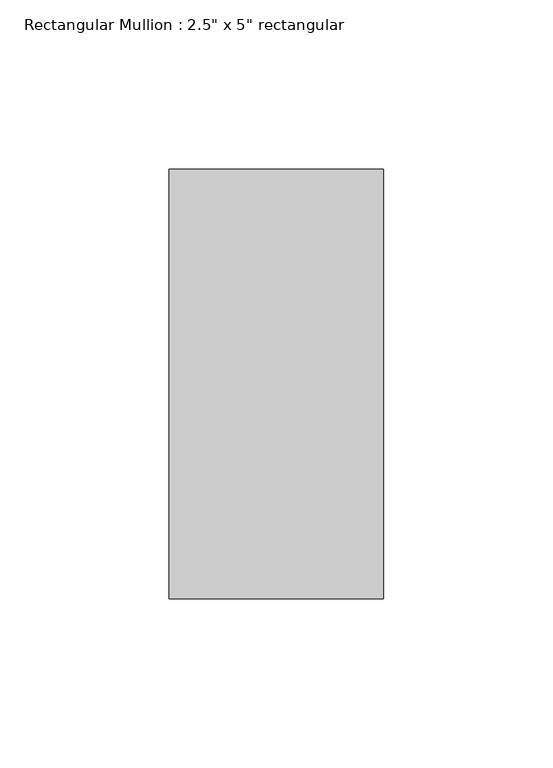
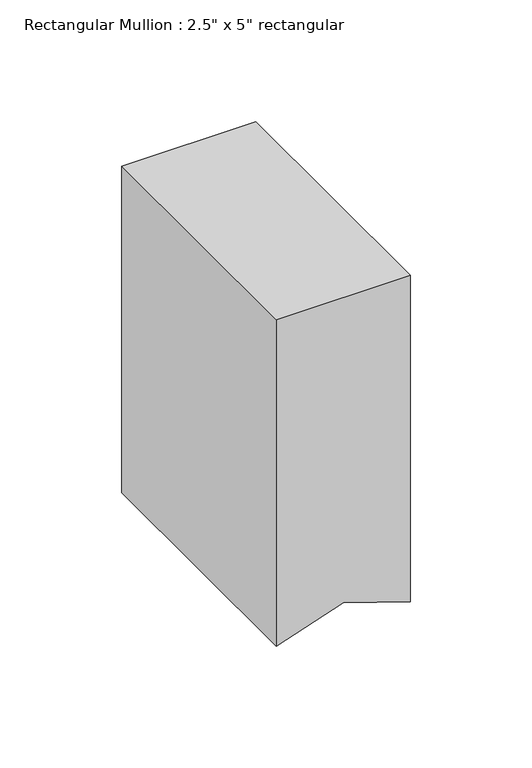
"""IFC4 building model written with IfcOpenShell, lengths in millimetres: member geometry."""

from ifc_helpers import new_model, si_unit, frame, origin, place, context, project, spatial, polyline, outline, extrude, source, transform, mapped, element, save


def member_f4359540(model_context):
    return source(origin(), model_context, "Body", "SweptSolid", [
        extrude(outline(polyline([(0.0, 31.75), (0.0, -31.75), (-163.7817895, -31.75), (-153.1984562, 0.0), (-163.7817895, 31.75), (0.0, 31.75)])), frame((0.0, -63.5, 0.0), z_axis=(0.0, 1.0, 0.0), x_axis=(0.0, 0.0, 1.0)), (0.0, 0.0, 1.0), 127.0),
    ])


if __name__ == "__main__":
    model = new_model("IFC4")
    model_context = context("Model", 3, world=origin())
    ifc_project = project(units=[si_unit("LENGTHUNIT", "METRE", prefix="MILLI")], contexts=[model_context])
    site = spatial("IfcSite", under=ifc_project)
    building = spatial("IfcBuilding", under=site)
    placement = place(None, origin())
    member_shape = member_f4359540(model_context)
    element("IfcMember", 1, ObjectType="Rectangular Mullion : 2.5\" x 5\" rectangular", at=placement, inside=building, context=model_context, shape_type="MappedRepresentation", body=[
        mapped(member_shape, transform((0.0, 0.0, 0.0), x_axis=(1.0, 0.0, 0.0), y_axis=(0.0, 1.0, 0.0), z_axis=(0.0, 0.0, 1.0))),
    ])
    save(model, "model.ifc")

# Revit data of these elements
# Type "Rectangular Mullion : 2.5\" x 5\" rectangular"
#   built-in parameter 1007304 = 0.416667 (stored number, unit not read)
#   built-in parameter 1007301 = 0.104167 (stored number, unit not read)
#   built-in parameter 1007300 = 0.104167 (stored number, unit not read)
# Element 1 (IfcMember, "Rectangular Mullion : 2.5\" x 5\" rectangular")
#   Materials on its faces: "Metal - Aluminum, Black-Annodized"
# Materials
#   "Metal - Aluminum, Black-Annodized": class "Metal", colour RGB 10 10 10, transparency 0, Cost = 0
